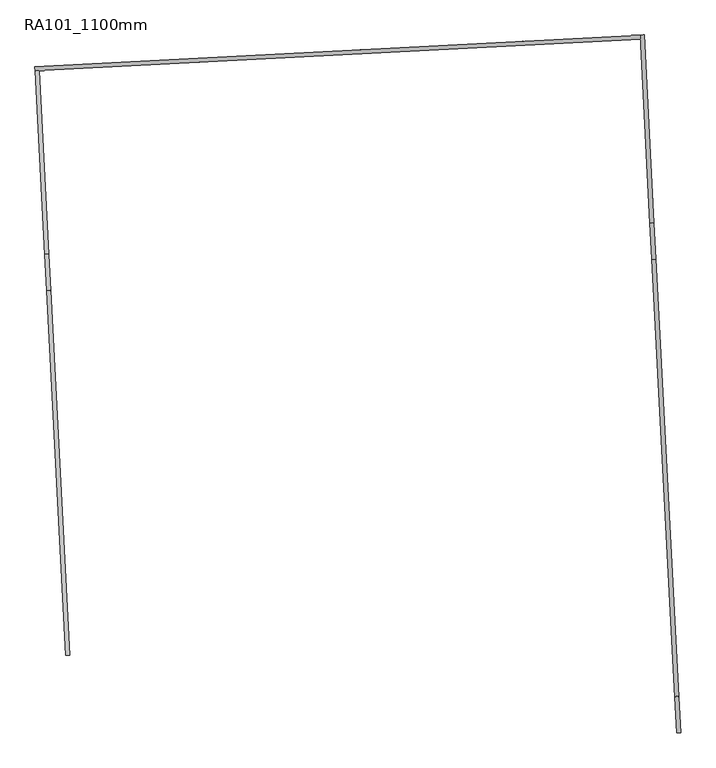
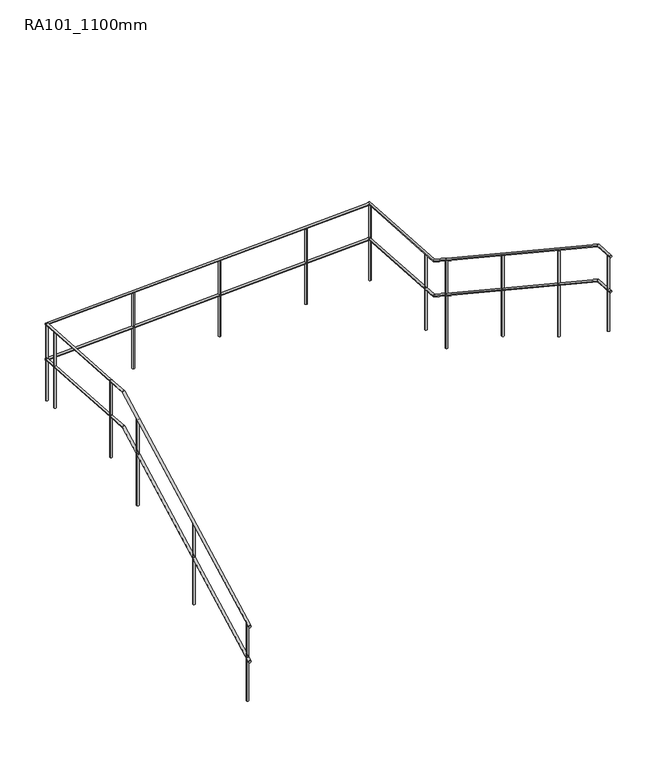
"""IFC4 building model written with IfcOpenShell, lengths in millimetres: railing geometry, RA101_1100mm."""

from ifc_helpers import new_model, si_unit, point, frame, frame_2d, origin, place, context, project, spatial, circle_curve, ellipse_curve, trimmed, segment, composite_curve, outline, extrude, source, transform, mapped, element, save
from ifc_brep_helpers import plane_surface, cylinder_surface, advanced_brep


def ra101_1100mm_925ff370(model_context):
    return source(origin(), model_context, "Body", "SolidModel", [
        advanced_brep(
        [(21553.8210897, 12464.3641407, 457.1248327), (21523.8622036, 12462.794062, 457.1248327), (21412.281847, 15165.0937775, 2210.0), (21382.3229609, 15163.5236988, 2210.0), (21398.3832997, 15430.2938589, 2210.0), (21368.4244136, 15428.7237802, 2210.0)],
        [
            (0, 1, ellipse_curve(frame((21538.8416467, 12463.5791013, 457.1248327), z_axis=(0.052335956242941364, -0.998629534754574, 0.0), x_axis=(0.0, 0.0, -1.0)), 17.8751673, 15.0)),
            (1, 0, ellipse_curve(frame((21538.8416467, 12463.5791013, 457.1248327), z_axis=(0.052335956242941364, -0.998629534754574, 0.0), x_axis=(0.0, 0.0, -1.0)), 17.8751673, 15.0)),
            (0, 2),
            (2, 3, ellipse_curve(frame((21397.302404, 15164.3087382, 2210.0), z_axis=(0.05018733030882, -0.957631309614881, -0.28359038545367027), x_axis=(-0.014841974004008681, 0.2832017346864693, -0.9589455111101147)), 15.6421818, 15.0)),
            (3, 1),
            (3, 2, ellipse_curve(frame((21397.302404, 15164.3087382, 2210.0), z_axis=(0.05018733030882, -0.957631309614881, -0.28359038545367027), x_axis=(-0.014841974004008681, 0.2832017346864693, -0.9589455111101147)), 15.6421818, 15.0)),
            (4, 5, circle_curve(frame((21383.4038566, 15429.5088195, 2210.0), z_axis=(-0.05233595624293373, 0.9986295347545745, 0.0), x_axis=(-0.9986295347545745, -0.05233595624293373, 0.0)), 15.0)),
            (5, 4, circle_curve(frame((21383.4038566, 15429.5088195, 2210.0), z_axis=(-0.05233595624293373, 0.9986295347545745, 0.0), x_axis=(-0.9986295347545745, -0.05233595624293373, 0.0)), 15.0)),
            (2, 4),
            (5, 3),
        ],
        [
            plane_surface(frame((21538.8416467, 12463.5791013, 475.0), z_axis=(0.052335956242941364, -0.998629534754574, 0.0), x_axis=(0.998629534754574, 0.052335956242941364, 0.0))),
            cylinder_surface(frame((21538.4146673, 12471.7263523, 462.4127052), z_axis=(0.04391787398555335, -0.8380029565528062, -0.5438954542495688), x_axis=(-0.998629534754574, -0.05233595624294136, 0.0)), 15.0),
            plane_surface(frame((21383.4038566, 15429.5088195, 2225.0), z_axis=(-0.05233595624293375, 0.9986295347545745, 0.0), x_axis=(0.9986295347545745, 0.05233595624293375, 0.0))),
            cylinder_surface(frame((21397.5345648, 15159.8788452, 2210.0), z_axis=(0.05233595624293373, -0.9986295347545745, 0.0), x_axis=(-0.9986295347545745, -0.05233595624293373, 0.0)), 15.0),
        ],
        [
            (0, [[1, 2]]),
            (1, [[-1, 3, 4, 5]]),
            (1, [[-2, -5, 6, -3]]),
            (2, [[7, 8]]),
            (3, [[-4, 9, -8, 10]]),
            (3, [[-6, -10, -7, -9]]),
        ],
    ),
        advanced_brep(
        [(21398.3832997, 15430.2938589, 2210.0), (21368.4244136, 15428.7237802, 2210.0), (21327.2273335, 16788.0305743, 2210.0), (21297.2684475, 16786.4604957, 2210.0)],
        [
            (0, 1, circle_curve(frame((21383.4038566, 15429.5088195, 2210.0), z_axis=(0.05233595624294149, -0.998629534754574, 0.0), x_axis=(-0.998629534754574, -0.05233595624294149, 0.0)), 15.0)),
            (1, 0, circle_curve(frame((21383.4038566, 15429.5088195, 2210.0), z_axis=(0.05233595624294149, -0.998629534754574, 0.0), x_axis=(-0.998629534754574, -0.05233595624294149, 0.0)), 15.0)),
            (2, 3, circle_curve(frame((21312.2478905, 16787.245535, 2210.0), z_axis=(-0.05233595624294149, 0.998629534754574, 0.0), x_axis=(-0.998629534754574, -0.05233595624294149, 0.0)), 15.0)),
            (3, 2, circle_curve(frame((21312.2478905, 16787.245535, 2210.0), z_axis=(-0.05233595624294149, 0.998629534754574, 0.0), x_axis=(-0.998629534754574, -0.05233595624294149, 0.0)), 15.0)),
            (0, 2),
            (3, 1),
        ],
        [
            plane_surface(frame((21383.4038566, 15429.5088195, 2225.0), z_axis=(0.05233595624294149, -0.998629534754574, 0.0), x_axis=(0.998629534754574, 0.05233595624294149, 0.0))),
            plane_surface(frame((21312.2478905, 16787.245535, 2225.0), z_axis=(-0.05233595624294221, 0.998629534754574, 0.0), x_axis=(0.998629534754574, 0.05233595624294221, 0.0))),
            cylinder_surface(frame((21383.4038566, 15429.5088195, 2210.0), z_axis=(0.05233595624294149, -0.998629534754574, 0.0), x_axis=(-0.998629534754574, -0.05233595624294149, 0.0)), 15.0),
        ],
        [
            (0, [[1, 2]]),
            (1, [[3, 4]]),
            (2, [[-1, 5, -4, 6]]),
            (2, [[-2, -6, -3, -5]]),
        ],
    ),
        advanced_brep(
        [(21297.2684475, 16786.4604957, 2210.0), (21295.6983688, 16816.4193817, 2210.0), (25777.8195811, 17021.2762305, 2210.0), (25776.2495024, 17051.2351166, 2210.0)],
        [
            (0, 1, circle_curve(frame((21296.4834082, 16801.4399387, 2210.0), z_axis=(-0.998629534754574, -0.05233595624294222, 0.0), x_axis=(-0.05233595624294222, 0.998629534754574, 0.0)), 15.0)),
            (1, 0, circle_curve(frame((21296.4834082, 16801.4399387, 2210.0), z_axis=(-0.998629534754574, -0.05233595624294222, 0.0), x_axis=(-0.05233595624294222, 0.998629534754574, 0.0)), 15.0)),
            (2, 3, circle_curve(frame((25777.0345417, 17036.2556736, 2210.0), z_axis=(0.998629534754574, 0.05233595624294222, 0.0), x_axis=(-0.05233595624294222, 0.998629534754574, 0.0)), 15.0)),
            (3, 2, circle_curve(frame((25777.0345417, 17036.2556736, 2210.0), z_axis=(0.998629534754574, 0.05233595624294222, 0.0), x_axis=(-0.05233595624294222, 0.998629534754574, 0.0)), 15.0)),
            (0, 2),
            (3, 1),
        ],
        [
            plane_surface(frame((21296.4834082, 16801.4399387, 2225.0), z_axis=(-0.998629534754574, -0.05233595624294149, 0.0), x_axis=(0.05233595624294149, -0.998629534754574, 0.0))),
            plane_surface(frame((25777.0345417, 17036.2556736, 2225.0), z_axis=(0.9986295347545739, 0.05233595624294333, 0.0), x_axis=(0.05233595624294333, -0.9986295347545739, 0.0))),
            cylinder_surface(frame((21296.4834082, 16801.4399387, 2210.0), z_axis=(-0.998629534754574, -0.05233595624294222, 0.0), x_axis=(-0.05233595624294222, 0.998629534754574, 0.0)), 15.0),
        ],
        [
            (0, [[1, 2]]),
            (1, [[3, 4]]),
            (2, [[-1, 5, -4, 6]]),
            (2, [[-2, -6, -3, -5]]),
        ],
    ),
        advanced_brep(
        [(25776.2495024, 17051.2351166, 2210.0), (25806.2083884, 17052.8051953, 2210.0), (25849.207708, 15659.1096221, 2210.0), (25879.1665941, 15660.6797008, 2210.0), (25863.1062554, 15393.9095407, 2382.1248327), (25893.0651414, 15395.4796194, 2382.1248327)],
        [
            (0, 1, circle_curve(frame((25791.2289454, 17052.0201559, 2210.0), z_axis=(-0.05233595624294333, 0.9986295347545739, 0.0), x_axis=(0.9986295347545739, 0.05233595624294333, 0.0)), 15.0)),
            (1, 0, circle_curve(frame((25791.2289454, 17052.0201559, 2210.0), z_axis=(-0.05233595624294333, 0.9986295347545739, 0.0), x_axis=(0.9986295347545739, 0.05233595624294333, 0.0)), 15.0)),
            (0, 2),
            (2, 3, ellipse_curve(frame((25864.1871511, 15659.8946614, 2210.0), z_axis=(-0.05018733030882886, 0.9576313096148807, -0.2835903854536695), x_axis=(-0.014841974004012624, 0.28320173468646914, 0.9589455111101145)), 15.6421818, 15.0)),
            (3, 1),
            (3, 2, ellipse_curve(frame((25864.1871511, 15659.8946614, 2210.0), z_axis=(-0.05018733030882886, 0.9576313096148807, -0.2835903854536695), x_axis=(-0.014841974004012624, 0.28320173468646914, 0.9589455111101145)), 15.6421818, 15.0)),
            (4, 5, ellipse_curve(frame((25878.0856984, 15394.69458, 2382.1248327), z_axis=(0.05233595624295016, -0.9986295347545736, 0.0), x_axis=(0.0, 0.0, -1.0)), 17.8751673, 15.0)),
            (5, 4, ellipse_curve(frame((25878.0856984, 15394.69458, 2382.1248327), z_axis=(0.05233595624295016, -0.9986295347545736, 0.0), x_axis=(0.0, 0.0, -1.0)), 17.8751673, 15.0)),
            (2, 4),
            (5, 3),
        ],
        [
            plane_surface(frame((25791.2289454, 17052.0201559, 2225.0), z_axis=(-0.05233595624294221, 0.998629534754574, 0.0), x_axis=(0.998629534754574, 0.05233595624294221, 0.0))),
            cylinder_surface(frame((25791.2289454, 17052.0201559, 2210.0), z_axis=(-0.05233595624294333, 0.9986295347545739, 0.0), x_axis=(0.9986295347545739, 0.05233595624294333, 0.0)), 15.0),
            plane_surface(frame((25878.0856984, 15394.69458, 2400.0), z_axis=(0.05233595624295016, -0.9986295347545736, 0.0), x_axis=(0.9986295347545736, 0.05233595624295016, 0.0))),
            cylinder_surface(frame((25864.3819695, 15656.1773035, 2212.4127052), z_axis=(-0.043917873985560775, 0.838002956552807, -0.5438954542495672), x_axis=(0.9986295347545737, 0.05233595624294905, 0.0)), 15.0),
        ],
        [
            (0, [[1, 2]]),
            (1, [[-1, 3, 4, 5]]),
            (1, [[-2, -5, 6, -3]]),
            (2, [[7, 8]]),
            (3, [[-4, 9, -8, 10]]),
            (3, [[-6, -10, -7, -9]]),
        ],
    ),
        advanced_brep(
        [(25863.1062554, 15393.9095407, 2382.1248327), (25893.0651414, 15395.4796194, 2382.1248327), (26032.9069145, 12153.9199551, 4485.0), (26062.8658005, 12155.4900338, 4485.0), (26046.8054618, 11888.7198737, 4485.0), (26076.7643478, 11890.2899524, 4485.0)],
        [
            (0, 1, ellipse_curve(frame((25878.0856984, 15394.69458, 2382.1248327), z_axis=(-0.052335956242941906, 0.998629534754574, 0.0), x_axis=(0.0, 0.0, -1.0)), 17.8751673, 15.0)),
            (1, 0, ellipse_curve(frame((25878.0856984, 15394.69458, 2382.1248327), z_axis=(-0.052335956242941906, 0.998629534754574, 0.0), x_axis=(0.0, 0.0, -1.0)), 17.8751673, 15.0)),
            (0, 2),
            (2, 3, ellipse_curve(frame((26047.8863575, 12154.7049944, 4485.0), z_axis=(-0.05018733030882246, 0.957631309614881, -0.28359038545366994), x_axis=(0.01484197400401534, -0.2832017346864691, -0.9589455111101146)), 15.6421818, 15.0)),
            (3, 1),
            (3, 2, ellipse_curve(frame((26047.8863575, 12154.7049944, 4485.0), z_axis=(-0.05018733030882246, 0.957631309614881, -0.28359038545366994), x_axis=(0.01484197400401534, -0.2832017346864691, -0.9589455111101146)), 15.6421818, 15.0)),
            (4, 5, circle_curve(frame((26061.7849048, 11889.5049131, 4485.0), z_axis=(0.05233595624293795, -0.9986295347545743, 0.0), x_axis=(0.9986295347545743, 0.05233595624293795, 0.0)), 15.0)),
            (5, 4, circle_curve(frame((26061.7849048, 11889.5049131, 4485.0), z_axis=(0.05233595624293795, -0.9986295347545743, 0.0), x_axis=(0.9986295347545743, 0.05233595624293795, 0.0)), 15.0)),
            (2, 4),
            (5, 3),
        ],
        [
            plane_surface(frame((25878.0856984, 15394.69458, 2400.0), z_axis=(-0.052335956242941906, 0.998629534754574, 0.0), x_axis=(0.998629534754574, 0.052335956242941906, 0.0))),
            cylinder_surface(frame((25878.5126777, 15386.5473291, 2387.4127052), z_axis=(-0.04391787398555386, 0.8380029565528069, -0.5438954542495675), x_axis=(0.998629534754574, 0.05233595624294191, 0.0)), 15.0),
            plane_surface(frame((26061.7849048, 11889.5049131, 4500.0), z_axis=(0.05233595624293795, -0.9986295347545743, 0.0), x_axis=(0.9986295347545743, 0.05233595624293795, 0.0))),
            cylinder_surface(frame((26047.6541966, 12159.1348874, 4485.0), z_axis=(-0.05233595624293795, 0.9986295347545743, 0.0), x_axis=(0.9986295347545743, 0.05233595624293795, 0.0)), 15.0),
        ],
        [
            (0, [[1, 2]]),
            (1, [[-1, 3, 4, 5]]),
            (1, [[-2, -5, 6, -3]]),
            (2, [[7, 8]]),
            (3, [[-4, 9, -8, 10]]),
            (3, [[-6, -10, -7, -9]]),
        ],
    ),
        advanced_brep(
        [(21553.8210897, 12464.3641407, 957.1248327), (21523.8622036, 12462.794062, 957.1248327), (21412.281847, 15165.0937775, 2710.0), (21382.3229609, 15163.5236988, 2710.0), (21398.3832997, 15430.2938589, 2710.0), (21368.4244136, 15428.7237802, 2710.0)],
        [
            (0, 1, ellipse_curve(frame((21538.8416467, 12463.5791013, 957.1248327), z_axis=(0.052335956242941364, -0.998629534754574, 0.0), x_axis=(0.0, 0.0, -1.0)), 17.8751673, 15.0)),
            (1, 0, ellipse_curve(frame((21538.8416467, 12463.5791013, 957.1248327), z_axis=(0.052335956242941364, -0.998629534754574, 0.0), x_axis=(0.0, 0.0, -1.0)), 17.8751673, 15.0)),
            (0, 2),
            (2, 3, ellipse_curve(frame((21397.302404, 15164.3087382, 2710.0), z_axis=(0.05018733030882, -0.957631309614881, -0.28359038545367027), x_axis=(-0.014841974004008681, 0.2832017346864693, -0.9589455111101147)), 15.6421818, 15.0)),
            (3, 1),
            (3, 2, ellipse_curve(frame((21397.302404, 15164.3087382, 2710.0), z_axis=(0.05018733030882, -0.957631309614881, -0.28359038545367027), x_axis=(-0.014841974004008681, 0.2832017346864693, -0.9589455111101147)), 15.6421818, 15.0)),
            (4, 5, circle_curve(frame((21383.4038566, 15429.5088195, 2710.0), z_axis=(-0.05233595624293373, 0.9986295347545745, 0.0), x_axis=(-0.9986295347545745, -0.05233595624293373, 0.0)), 15.0)),
            (5, 4, circle_curve(frame((21383.4038566, 15429.5088195, 2710.0), z_axis=(-0.05233595624293373, 0.9986295347545745, 0.0), x_axis=(-0.9986295347545745, -0.05233595624293373, 0.0)), 15.0)),
            (2, 4),
            (5, 3),
        ],
        [
            plane_surface(frame((21538.8416467, 12463.5791013, 975.0), z_axis=(0.052335956242941364, -0.998629534754574, 0.0), x_axis=(0.998629534754574, 0.052335956242941364, 0.0))),
            cylinder_surface(frame((21538.4146673, 12471.7263523, 962.4127052), z_axis=(0.04391787398555335, -0.8380029565528062, -0.5438954542495688), x_axis=(-0.998629534754574, -0.05233595624294136, 0.0)), 15.0),
            plane_surface(frame((21383.4038566, 15429.5088195, 2725.0), z_axis=(-0.05233595624293375, 0.9986295347545745, 0.0), x_axis=(0.9986295347545745, 0.05233595624293375, 0.0))),
            cylinder_surface(frame((21397.5345648, 15159.8788452, 2710.0), z_axis=(0.05233595624293373, -0.9986295347545745, 0.0), x_axis=(-0.9986295347545745, -0.05233595624293373, 0.0)), 15.0),
        ],
        [
            (0, [[1, 2]]),
            (1, [[-1, 3, 4, 5]]),
            (1, [[-2, -5, 6, -3]]),
            (2, [[7, 8]]),
            (3, [[-4, 9, -8, 10]]),
            (3, [[-6, -10, -7, -9]]),
        ],
    ),
        advanced_brep(
        [(21398.3832997, 15430.2938589, 2710.0), (21368.4244136, 15428.7237802, 2710.0), (21327.2273335, 16788.0305743, 2710.0), (21297.2684475, 16786.4604957, 2710.0)],
        [
            (0, 1, circle_curve(frame((21383.4038566, 15429.5088195, 2710.0), z_axis=(0.05233595624294149, -0.998629534754574, 0.0), x_axis=(-0.998629534754574, -0.05233595624294149, 0.0)), 15.0)),
            (1, 0, circle_curve(frame((21383.4038566, 15429.5088195, 2710.0), z_axis=(0.05233595624294149, -0.998629534754574, 0.0), x_axis=(-0.998629534754574, -0.05233595624294149, 0.0)), 15.0)),
            (2, 3, circle_curve(frame((21312.2478905, 16787.245535, 2710.0), z_axis=(-0.05233595624294149, 0.998629534754574, 0.0), x_axis=(-0.998629534754574, -0.05233595624294149, 0.0)), 15.0)),
            (3, 2, circle_curve(frame((21312.2478905, 16787.245535, 2710.0), z_axis=(-0.05233595624294149, 0.998629534754574, 0.0), x_axis=(-0.998629534754574, -0.05233595624294149, 0.0)), 15.0)),
            (0, 2),
            (3, 1),
        ],
        [
            plane_surface(frame((21383.4038566, 15429.5088195, 2725.0), z_axis=(0.05233595624294149, -0.998629534754574, 0.0), x_axis=(0.998629534754574, 0.05233595624294149, 0.0))),
            plane_surface(frame((21312.2478905, 16787.245535, 2725.0), z_axis=(-0.05233595624294221, 0.998629534754574, 0.0), x_axis=(0.998629534754574, 0.05233595624294221, 0.0))),
            cylinder_surface(frame((21383.4038566, 15429.5088195, 2710.0), z_axis=(0.05233595624294149, -0.998629534754574, 0.0), x_axis=(-0.998629534754574, -0.05233595624294149, 0.0)), 15.0),
        ],
        [
            (0, [[1, 2]]),
            (1, [[3, 4]]),
            (2, [[-1, 5, -4, 6]]),
            (2, [[-2, -6, -3, -5]]),
        ],
    ),
        advanced_brep(
        [(21297.2684475, 16786.4604957, 2710.0), (21295.6983688, 16816.4193817, 2710.0), (25777.8195811, 17021.2762305, 2710.0), (25776.2495024, 17051.2351166, 2710.0)],
        [
            (0, 1, circle_curve(frame((21296.4834082, 16801.4399387, 2710.0), z_axis=(-0.998629534754574, -0.05233595624294222, 0.0), x_axis=(-0.05233595624294222, 0.998629534754574, 0.0)), 15.0)),
            (1, 0, circle_curve(frame((21296.4834082, 16801.4399387, 2710.0), z_axis=(-0.998629534754574, -0.05233595624294222, 0.0), x_axis=(-0.05233595624294222, 0.998629534754574, 0.0)), 15.0)),
            (2, 3, circle_curve(frame((25777.0345417, 17036.2556736, 2710.0), z_axis=(0.998629534754574, 0.05233595624294222, 0.0), x_axis=(-0.05233595624294222, 0.998629534754574, 0.0)), 15.0)),
            (3, 2, circle_curve(frame((25777.0345417, 17036.2556736, 2710.0), z_axis=(0.998629534754574, 0.05233595624294222, 0.0), x_axis=(-0.05233595624294222, 0.998629534754574, 0.0)), 15.0)),
            (0, 2),
            (3, 1),
        ],
        [
            plane_surface(frame((21296.4834082, 16801.4399387, 2725.0), z_axis=(-0.998629534754574, -0.05233595624294149, 0.0), x_axis=(0.05233595624294149, -0.998629534754574, 0.0))),
            plane_surface(frame((25777.0345417, 17036.2556736, 2725.0), z_axis=(0.9986295347545739, 0.05233595624294333, 0.0), x_axis=(0.05233595624294333, -0.9986295347545739, 0.0))),
            cylinder_surface(frame((21296.4834082, 16801.4399387, 2710.0), z_axis=(-0.998629534754574, -0.05233595624294222, 0.0), x_axis=(-0.05233595624294222, 0.998629534754574, 0.0)), 15.0),
        ],
        [
            (0, [[1, 2]]),
            (1, [[3, 4]]),
            (2, [[-1, 5, -4, 6]]),
            (2, [[-2, -6, -3, -5]]),
        ],
    ),
        advanced_brep(
        [(25776.2495024, 17051.2351166, 2710.0), (25806.2083884, 17052.8051953, 2710.0), (25849.207708, 15659.1096221, 2710.0), (25879.1665941, 15660.6797008, 2710.0), (25863.1062554, 15393.9095407, 2882.1248327), (25893.0651414, 15395.4796194, 2882.1248327)],
        [
            (0, 1, circle_curve(frame((25791.2289454, 17052.0201559, 2710.0), z_axis=(-0.05233595624294333, 0.9986295347545739, 0.0), x_axis=(0.9986295347545739, 0.05233595624294333, 0.0)), 15.0)),
            (1, 0, circle_curve(frame((25791.2289454, 17052.0201559, 2710.0), z_axis=(-0.05233595624294333, 0.9986295347545739, 0.0), x_axis=(0.9986295347545739, 0.05233595624294333, 0.0)), 15.0)),
            (0, 2),
            (2, 3, ellipse_curve(frame((25864.1871511, 15659.8946614, 2710.0), z_axis=(-0.05018733030882886, 0.9576313096148807, -0.2835903854536695), x_axis=(-0.014841974004012624, 0.28320173468646914, 0.9589455111101145)), 15.6421818, 15.0)),
            (3, 1),
            (3, 2, ellipse_curve(frame((25864.1871511, 15659.8946614, 2710.0), z_axis=(-0.05018733030882886, 0.9576313096148807, -0.2835903854536695), x_axis=(-0.014841974004012624, 0.28320173468646914, 0.9589455111101145)), 15.6421818, 15.0)),
            (4, 5, ellipse_curve(frame((25878.0856984, 15394.69458, 2882.1248327), z_axis=(0.05233595624295016, -0.9986295347545736, 0.0), x_axis=(0.0, 0.0, -1.0)), 17.8751673, 15.0)),
            (5, 4, ellipse_curve(frame((25878.0856984, 15394.69458, 2882.1248327), z_axis=(0.05233595624295016, -0.9986295347545736, 0.0), x_axis=(0.0, 0.0, -1.0)), 17.8751673, 15.0)),
            (2, 4),
            (5, 3),
        ],
        [
            plane_surface(frame((25791.2289454, 17052.0201559, 2725.0), z_axis=(-0.05233595624294221, 0.998629534754574, 0.0), x_axis=(0.998629534754574, 0.05233595624294221, 0.0))),
            cylinder_surface(frame((25791.2289454, 17052.0201559, 2710.0), z_axis=(-0.05233595624294333, 0.9986295347545739, 0.0), x_axis=(0.9986295347545739, 0.05233595624294333, 0.0)), 15.0),
            plane_surface(frame((25878.0856984, 15394.69458, 2900.0), z_axis=(0.05233595624295016, -0.9986295347545736, 0.0), x_axis=(0.9986295347545736, 0.05233595624295016, 0.0))),
            cylinder_surface(frame((25864.3819695, 15656.1773035, 2712.4127052), z_axis=(-0.043917873985560775, 0.838002956552807, -0.5438954542495672), x_axis=(0.9986295347545737, 0.05233595624294905, 0.0)), 15.0),
        ],
        [
            (0, [[1, 2]]),
            (1, [[-1, 3, 4, 5]]),
            (1, [[-2, -5, 6, -3]]),
            (2, [[7, 8]]),
            (3, [[-4, 9, -8, 10]]),
            (3, [[-6, -10, -7, -9]]),
        ],
    ),
        advanced_brep(
        [(25863.1062554, 15393.9095407, 2882.1248327), (25893.0651414, 15395.4796194, 2882.1248327), (26032.9069145, 12153.9199551, 4985.0), (26062.8658005, 12155.4900338, 4985.0), (26046.8054618, 11888.7198737, 4985.0), (26076.7643478, 11890.2899524, 4985.0)],
        [
            (0, 1, ellipse_curve(frame((25878.0856984, 15394.69458, 2882.1248327), z_axis=(-0.052335956242941906, 0.998629534754574, 0.0), x_axis=(0.0, 0.0, -1.0)), 17.8751673, 15.0)),
            (1, 0, ellipse_curve(frame((25878.0856984, 15394.69458, 2882.1248327), z_axis=(-0.052335956242941906, 0.998629534754574, 0.0), x_axis=(0.0, 0.0, -1.0)), 17.8751673, 15.0)),
            (0, 2),
            (2, 3, ellipse_curve(frame((26047.8863575, 12154.7049944, 4985.0), z_axis=(-0.05018733030882246, 0.957631309614881, -0.28359038545366994), x_axis=(0.01484197400401534, -0.2832017346864691, -0.9589455111101146)), 15.6421818, 15.0)),
            (3, 1),
            (3, 2, ellipse_curve(frame((26047.8863575, 12154.7049944, 4985.0), z_axis=(-0.05018733030882246, 0.957631309614881, -0.28359038545366994), x_axis=(0.01484197400401534, -0.2832017346864691, -0.9589455111101146)), 15.6421818, 15.0)),
            (4, 5, circle_curve(frame((26061.7849048, 11889.5049131, 4985.0), z_axis=(0.05233595624293795, -0.9986295347545743, 0.0), x_axis=(0.9986295347545743, 0.05233595624293795, 0.0)), 15.0)),
            (5, 4, circle_curve(frame((26061.7849048, 11889.5049131, 4985.0), z_axis=(0.05233595624293795, -0.9986295347545743, 0.0), x_axis=(0.9986295347545743, 0.05233595624293795, 0.0)), 15.0)),
            (2, 4),
            (5, 3),
        ],
        [
            plane_surface(frame((25878.0856984, 15394.69458, 2900.0), z_axis=(-0.052335956242941906, 0.998629534754574, 0.0), x_axis=(0.998629534754574, 0.052335956242941906, 0.0))),
            cylinder_surface(frame((25878.5126777, 15386.5473291, 2887.4127052), z_axis=(-0.04391787398555386, 0.8380029565528069, -0.5438954542495675), x_axis=(0.998629534754574, 0.05233595624294191, 0.0)), 15.0),
            plane_surface(frame((26061.7849048, 11889.5049131, 5000.0), z_axis=(0.05233595624293795, -0.9986295347545743, 0.0), x_axis=(0.9986295347545743, 0.05233595624293795, 0.0))),
            cylinder_surface(frame((26047.6541966, 12159.1348874, 4985.0), z_axis=(-0.05233595624293795, 0.9986295347545743, 0.0), x_axis=(0.9986295347545743, 0.05233595624293795, 0.0)), 15.0),
        ],
        [
            (0, [[1, 2]]),
            (1, [[-1, 3, 4, 5]]),
            (1, [[-2, -5, 6, -3]]),
            (2, [[7, 8]]),
            (3, [[-4, 9, -8, 10]]),
            (3, [[-6, -10, -7, -9]]),
        ],
    ),
        extrude(outline(composite_curve([segment(trimmed(circle_curve(frame_2d((26003.6919934, 12997.9836966)), 15.0), [point((26018.6714364, 12998.768736))], [point((25988.7125504, 12997.1986573))], False, "CARTESIAN"), True, "CONTINUOUS"), segment(trimmed(circle_curve(frame_2d((26003.6919934, 12997.9836966)), 15.0), [point((25988.7125504, 12997.1986573))], [point((26018.6714364, 12998.768736))], False, "CARTESIAN"), True, "CONTINUOUS")], self_intersect=False)), frame((0.0, 0.0, 3200.0), z_axis=(0.0, 0.0, 1.0), x_axis=(1.0, 0.0, 0.0)), (0.0, 0.0, 1.0), 1225.5555556),
        extrude(outline(composite_curve([segment(trimmed(circle_curve(frame_2d((25940.8888459, 14196.3391383)), 15.0), [point((25955.8682889, 14197.1241777))], [point((25925.9094029, 14195.554099))], False, "CARTESIAN"), True, "CONTINUOUS"), segment(trimmed(circle_curve(frame_2d((25940.8888459, 14196.3391383)), 15.0), [point((25925.9094029, 14195.554099))], [point((25955.8682889, 14197.1241777))], False, "CARTESIAN"), True, "CONTINUOUS")], self_intersect=False)), frame((0.0, 0.0, 2500.0), z_axis=(0.0, 0.0, 1.0), x_axis=(1.0, 0.0, 0.0)), (0.0, 0.0, 1.0), 1147.7777778),
        extrude(outline(composite_curve([segment(trimmed(circle_curve(frame_2d((25854.8171323, 15838.6852712)), 15.0), [point((25869.7965753, 15839.4703105))], [point((25839.8376892, 15837.9002318))], False, "CARTESIAN"), True, "CONTINUOUS"), segment(trimmed(circle_curve(frame_2d((25854.8171323, 15838.6852712)), 15.0), [point((25839.8376892, 15837.9002318))], [point((25869.7965753, 15839.4703105))], False, "CARTESIAN"), True, "CONTINUOUS")], self_intersect=False)), frame((0.0, 0.0, 1625.0), z_axis=(0.0, 0.0, 1.0), x_axis=(1.0, 0.0, 0.0)), (0.0, 0.0, 1.0), 1070.0),
        extrude(outline(composite_curve([segment(trimmed(circle_curve(frame_2d((24906.5291763, 16990.6344205)), 15.0), [point((24905.744137, 17005.6138635))], [point((24907.3142156, 16975.6549775))], False, "CARTESIAN"), True, "CONTINUOUS"), segment(trimmed(circle_curve(frame_2d((24906.5291763, 16990.6344205)), 15.0), [point((24907.3142156, 16975.6549775))], [point((24905.744137, 17005.6138635))], False, "CARTESIAN"), True, "CONTINUOUS")], self_intersect=False)), frame((0.0, 0.0, 1625.0), z_axis=(0.0, 0.0, 1.0), x_axis=(1.0, 0.0, 0.0)), (0.0, 0.0, 1.0), 1070.0),
        extrude(outline(composite_curve([segment(trimmed(circle_curve(frame_2d((23708.1737346, 16927.831273)), 15.0), [point((23707.3886952, 16942.810716))], [point((23708.9587739, 16912.85183))], False, "CARTESIAN"), True, "CONTINUOUS"), segment(trimmed(circle_curve(frame_2d((23708.1737346, 16927.831273)), 15.0), [point((23708.9587739, 16912.85183))], [point((23707.3886952, 16942.810716))], False, "CARTESIAN"), True, "CONTINUOUS")], self_intersect=False)), frame((0.0, 0.0, 1625.0), z_axis=(0.0, 0.0, 1.0), x_axis=(1.0, 0.0, 0.0)), (0.0, 0.0, 1.0), 1070.0),
        extrude(outline(composite_curve([segment(trimmed(circle_curve(frame_2d((22509.8182929, 16865.0281255)), 15.0), [point((22509.0332535, 16880.0075685))], [point((22510.6033322, 16850.0486825))], False, "CARTESIAN"), True, "CONTINUOUS"), segment(trimmed(circle_curve(frame_2d((22509.8182929, 16865.0281255)), 15.0), [point((22510.6033322, 16850.0486825))], [point((22509.0332535, 16880.0075685))], False, "CARTESIAN"), True, "CONTINUOUS")], self_intersect=False)), frame((0.0, 0.0, 1625.0), z_axis=(0.0, 0.0, 1.0), x_axis=(1.0, 0.0, 0.0)), (0.0, 0.0, 1.0), 1070.0),
        extrude(outline(composite_curve([segment(trimmed(circle_curve(frame_2d((21320.6007091, 16627.8642613)), 15.0), [point((21305.6212661, 16627.0792219))], [point((21335.5801522, 16628.6493006))], False, "CARTESIAN"), True, "CONTINUOUS"), segment(trimmed(circle_curve(frame_2d((21320.6007091, 16627.8642613)), 15.0), [point((21335.5801522, 16628.6493006))], [point((21305.6212661, 16627.0792219))], False, "CARTESIAN"), True, "CONTINUOUS")], self_intersect=False)), frame((0.0, 0.0, 1625.0), z_axis=(0.0, 0.0, 1.0), x_axis=(1.0, 0.0, 0.0)), (0.0, 0.0, 1.0), 1070.0),
        extrude(outline(composite_curve([segment(trimmed(circle_curve(frame_2d((21413.2353517, 14860.2899847)), 15.0), [point((21398.2559087, 14859.5049454))], [point((21428.2147947, 14861.0750241))], False, "CARTESIAN"), True, "CONTINUOUS"), segment(trimmed(circle_curve(frame_2d((21413.2353517, 14860.2899847)), 15.0), [point((21428.2147947, 14861.0750241))], [point((21398.2559087, 14859.5049454))], False, "CARTESIAN"), True, "CONTINUOUS")], self_intersect=False)), frame((0.0, 0.0, 1275.0), z_axis=(0.0, 0.0, 1.0), x_axis=(1.0, 0.0, 0.0)), (0.0, 0.0, 1.0), 1225.5555556),
        extrude(outline(composite_curve([segment(trimmed(circle_curve(frame_2d((21476.0384992, 13661.934543)), 15.0), [point((21461.0590562, 13661.1495037))], [point((21491.0179422, 13662.7195824))], False, "CARTESIAN"), True, "CONTINUOUS"), segment(trimmed(circle_curve(frame_2d((21476.0384992, 13661.934543)), 15.0), [point((21491.0179422, 13662.7195824))], [point((21461.0590562, 13661.1495037))], False, "CARTESIAN"), True, "CONTINUOUS")], self_intersect=False)), frame((0.0, 0.0, 575.0), z_axis=(0.0, 0.0, 1.0), x_axis=(1.0, 0.0, 0.0)), (0.0, 0.0, 1.0), 1147.7777778),
        extrude(outline(composite_curve([segment(trimmed(circle_curve(frame_2d((25878.0856984, 15394.69458)), 15.0), [point((25893.0651414, 15395.4796194))], [point((25863.1062554, 15393.9095407))], False, "CARTESIAN"), True, "CONTINUOUS"), segment(trimmed(circle_curve(frame_2d((25878.0856984, 15394.69458)), 15.0), [point((25863.1062554, 15393.9095407))], [point((25893.0651414, 15395.4796194))], False, "CARTESIAN"), True, "CONTINUOUS")], self_intersect=False)), frame((0.0, 0.0, 1625.0), z_axis=(0.0, 0.0, 1.0), x_axis=(1.0, 0.0, 0.0)), (0.0, 0.0, 1.0), 1245.0),
        extrude(outline(composite_curve([segment(trimmed(circle_curve(frame_2d((25792.0139848, 17037.0407129)), 15.0), [point((25791.2289454, 17052.0201559))], [point((25792.7990241, 17022.0612699))], False, "CARTESIAN"), True, "CONTINUOUS"), segment(trimmed(circle_curve(frame_2d((25792.0139848, 17037.0407129)), 15.0), [point((25792.7990241, 17022.0612699))], [point((25791.2289454, 17052.0201559))], False, "CARTESIAN"), True, "CONTINUOUS")], self_intersect=False)), frame((0.0, 0.0, 1625.0), z_axis=(0.0, 0.0, 1.0), x_axis=(1.0, 0.0, 0.0)), (0.0, 0.0, 1.0), 1070.0),
        extrude(outline(composite_curve([segment(trimmed(circle_curve(frame_2d((21311.4628512, 16802.224978)), 15.0), [point((21296.4834082, 16801.4399387))], [point((21326.4422942, 16803.0100174))], False, "CARTESIAN"), True, "CONTINUOUS"), segment(trimmed(circle_curve(frame_2d((21311.4628512, 16802.224978)), 15.0), [point((21326.4422942, 16803.0100174))], [point((21296.4834082, 16801.4399387))], False, "CARTESIAN"), True, "CONTINUOUS")], self_intersect=False)), frame((0.0, 0.0, 1625.0), z_axis=(0.0, 0.0, 1.0), x_axis=(1.0, 0.0, 0.0)), (0.0, 0.0, 1.0), 1070.0),
        extrude(outline(composite_curve([segment(trimmed(circle_curve(frame_2d((21383.4038566, 15429.5088195)), 15.0), [point((21368.4244136, 15428.7237802))], [point((21398.3832997, 15430.2938589))], False, "CARTESIAN"), True, "CONTINUOUS"), segment(trimmed(circle_curve(frame_2d((21383.4038566, 15429.5088195)), 15.0), [point((21398.3832997, 15430.2938589))], [point((21368.4244136, 15428.7237802))], False, "CARTESIAN"), True, "CONTINUOUS")], self_intersect=False)), frame((0.0, 0.0, 1625.0), z_axis=(0.0, 0.0, 1.0), x_axis=(1.0, 0.0, 0.0)), (0.0, 0.0, 1.0), 1070.0),
        extrude(outline(composite_curve([segment(trimmed(circle_curve(frame_2d((26059.168107, 11939.4363898)), 15.0), [point((26074.14755, 11940.2214291))], [point((26044.188664, 11938.6513504))], False, "CARTESIAN"), True, "CONTINUOUS"), segment(trimmed(circle_curve(frame_2d((26059.168107, 11939.4363898)), 15.0), [point((26044.188664, 11938.6513504))], [point((26074.14755, 11940.2214291))], False, "CARTESIAN"), True, "CONTINUOUS")], self_intersect=False)), frame((0.0, 0.0, 3900.0), z_axis=(0.0, 0.0, 1.0), x_axis=(1.0, 0.0, 0.0)), (0.0, 0.0, 1.0), 1070.0),
        extrude(outline(composite_curve([segment(trimmed(circle_curve(frame_2d((21536.2248489, 12513.5105781)), 15.0), [point((21521.2454058, 12512.7255387))], [point((21551.2042919, 12514.2956174))], False, "CARTESIAN"), True, "CONTINUOUS"), segment(trimmed(circle_curve(frame_2d((21536.2248489, 12513.5105781)), 15.0), [point((21551.2042919, 12514.2956174))], [point((21521.2454058, 12512.7255387))], False, "CARTESIAN"), True, "CONTINUOUS")], self_intersect=False)), frame((0.0, 0.0, -125.0), z_axis=(0.0, 0.0, 1.0), x_axis=(1.0, 0.0, 0.0)), (0.0, 0.0, 1.0), 1102.4074074),
    ])


if __name__ == "__main__":
    model = new_model("IFC4")
    model_context = context("Model", 3, world=origin())
    ifc_project = project(units=[si_unit("LENGTHUNIT", "METRE", prefix="MILLI")], contexts=[model_context])
    site = spatial("IfcSite", under=ifc_project)
    building = spatial("IfcBuilding", under=site)
    placement = place(None, origin())
    ra101_1100mm_shape = ra101_1100mm_925ff370(model_context)
    element("IfcRailing", 1, ObjectType="RA101_1100mm", at=placement, inside=building, context=model_context, shape_type="MappedRepresentation", body=[
        mapped(ra101_1100mm_shape, transform((0.0, 0.0, 0.0), x_axis=(1.0, 0.0, 0.0), y_axis=(0.0, 1.0, 0.0), z_axis=(0.0, 0.0, 1.0))),
    ])
    save(model, "model.ifc")
